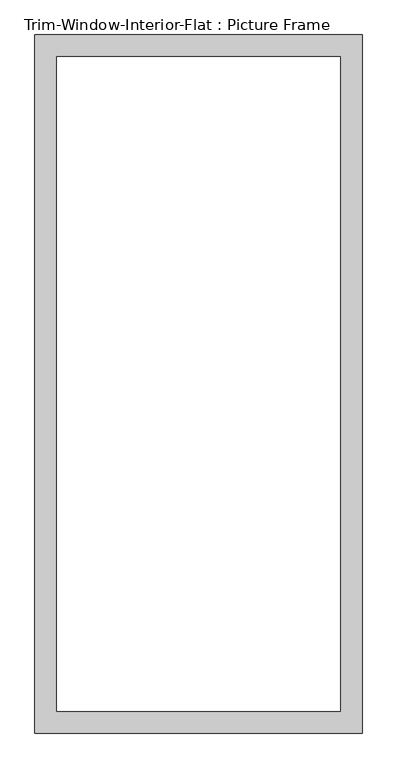
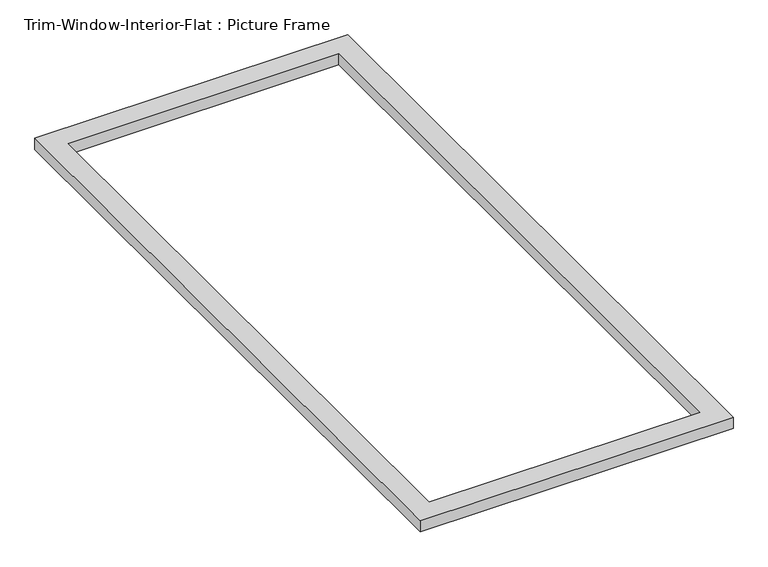
"""IFC4 building model written with IfcOpenShell, lengths in millimetres: proxy geometry, Trim-Window-Interior-Flat : Picture Frame."""

from ifc_helpers import new_model, si_unit, origin, origin_with_axes, place, context, project, spatial, polyline, outline, extrude, source, transform, mapped, element, save


def trim_window_interior_flat_picture_frame_f957ae71(model_context):
    return source(origin(), model_context, "Body", "SweptSolid", [
        extrude(outline(polyline([(425.45, 44.45), (425.45, -1771.65), (-425.45, -1771.65), (-425.45, 44.45), (425.45, 44.45)]), holes=[polyline([(368.3, -12.7), (-368.3, -12.7), (-368.3, -1714.5), (368.3, -1714.5), (368.3, -12.7)])]), origin_with_axes(), (0.0, 0.0, 1.0), 31.75),
    ])


if __name__ == "__main__":
    model = new_model("IFC4")
    model_context = context("Model", 3, world=origin())
    ifc_project = project(units=[si_unit("LENGTHUNIT", "METRE", prefix="MILLI")], contexts=[model_context])
    site = spatial("IfcSite", under=ifc_project)
    building = spatial("IfcBuilding", under=site)
    placement = place(None, origin())
    trim_window_interior_flat_picture_frame_shape = trim_window_interior_flat_picture_frame_f957ae71(model_context)
    element("IfcBuildingElementProxy", 1, Name="Trim-Window-Interior-Flat : Picture Frame", ObjectType="Trim-Window-Interior-Flat : Picture Frame", at=placement, inside=building, context=model_context, shape_type="MappedRepresentation", body=[
        mapped(trim_window_interior_flat_picture_frame_shape, transform((0.0, 0.0, 0.0), x_axis=(1.0, 0.0, 0.0), y_axis=(0.0, 1.0, 0.0), z_axis=(0.0, 0.0, 1.0))),
    ])
    save(model, "model.ifc")

# Revit data of these elements
# Type "Trim-Window-Interior-Flat : Picture Frame"
#   Trim Thickness_Picture Frame = 0' - 1 1/4"
#   Trim Width = 0' - 2 1/4"
#   Trim Thickness_with Sill = 0' - 0 3/4"
#   Sill Thickness = 0' - 1 1/4"
#   Opening Width [instance default] = 2' - 0"
#   Opening Height [instance default] = 3' - 0"
#   Default Elevation = 4' - 0"
#   Sill = no
#   Picture Frame = yes
#   Trim Material [instance default] = none
# Element 1 (IfcBuildingElementProxy, "Trim-Window-Interior-Flat : Picture Frame")
#   Opening Width = 2' - 6"
#   Opening Height = 5' - 8"
#   Trim Material = 1X WOOD COMPOSITE TRIM
#   Materials on its faces: "1X WOOD COMPOSITE TRIM"
# Materials
#   "1X WOOD COMPOSITE TRIM": class "Generic", colour RGB 88 61 61, transparency 0, Cost = 0
